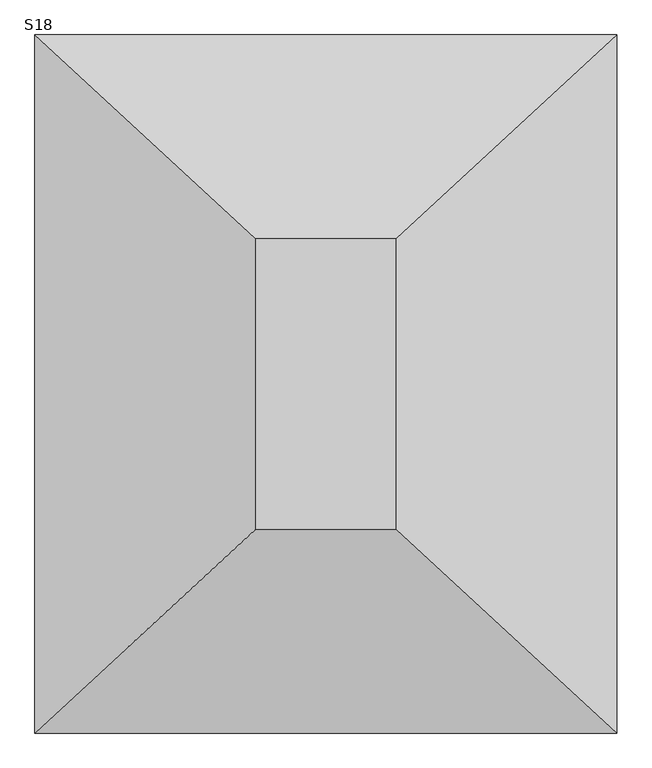
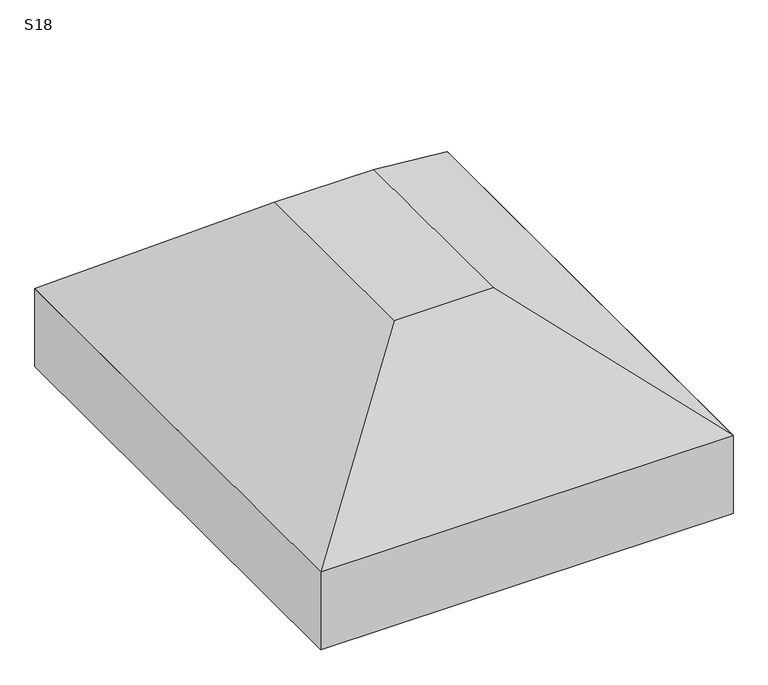
"""IFC4 building model written with IfcOpenShell, lengths in millimetres: fastener geometry, TQS - Sapata : S18."""

from ifc_helpers import new_model, si_unit, frame, origin, place, context, project, spatial, polyline, outline, extrude, faceted_brep, source, transform, mapped, element, save


def s18_084f9c6a(model_context):
    return source(origin(), model_context, "Body", "SolidModel", [
        faceted_brep([(-80.0, 50.0, 0.0), (-320.0, 50.0, 0.0), (-320.0, -450.0, 0.0), (-80.0, -450.0, 0.0), (300.0, 400.0, -300.0), (300.0, -800.0, -300.0), (-700.0, -800.0, -300.0), (-700.0, 400.0, -300.0)], [[[0, 1, 2, 3]], [[4, 5, 6, 7]], [[4, 7, 1, 0]], [[7, 6, 2, 1]], [[6, 5, 3, 2]], [[5, 4, 0, 3]]]),
        extrude(outline(polyline([(300.0, 400.0), (300.0, -800.0), (-700.0, -800.0), (-700.0, 400.0), (300.0, 400.0)])), frame((0.0, 0.0, -500.0), z_axis=(0.0, 0.0, 1.0), x_axis=(1.0, 0.0, 0.0)), (0.0, 0.0, 1.0), 200.0),
    ])


if __name__ == "__main__":
    model = new_model("IFC4")
    model_context = context("Model", 3, world=origin())
    ifc_project = project(units=[si_unit("LENGTHUNIT", "METRE", prefix="MILLI")], contexts=[model_context])
    site = spatial("IfcSite", under=ifc_project)
    building = spatial("IfcBuilding", under=site)
    placement = place(None, origin())
    s18_shape = s18_084f9c6a(model_context)
    element("IfcFastener", 1, ObjectType="TQS - Sapata : S18", at=placement, inside=building, context=model_context, shape_type="MappedRepresentation", body=[
        mapped(s18_shape, transform((0.0, 0.0, 0.0), x_axis=(1.0, 0.0, 0.0), y_axis=(0.0, 1.0, 0.0), z_axis=(0.0, 0.0, 1.0))),
    ])
    save(model, "model.ifc")

# Revit data of these elements
# Type "TQS - Sapata : S18"
#   TY = 0.50 m
#   TX = 0.24 m
#   HS = 0.50 m
#   H0 = 0.20 m
#   EXCYABS = 0.60 m
#   EXCY = 0.00 m
#   EXCXABS = 0.50 m
#   EXCX = 0.00 m
#   DIMY = 1.20 m
#   DIMX = 1.00 m
#   Material estrutural = Concreto - Concreto concretado no local
#   Width = 0
#   Length = 0
# Element 1 (IfcFastener, "TQS - Sapata : S18")
#   Materials on its faces: "Concreto - Concreto concretado no local"
# Materials
#   "Concreto - Concreto concretado no local": class "Concreto", colour RGB 192 192 192, transparency 0
